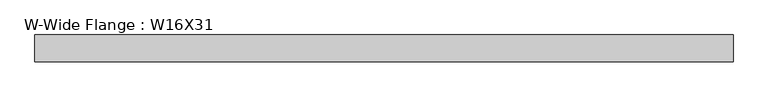
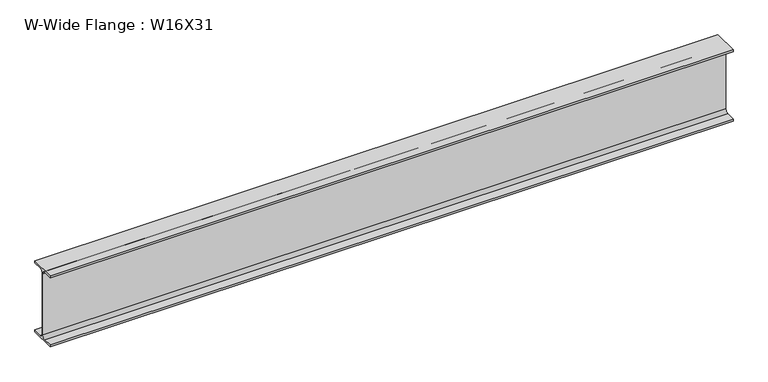
"""IFC4 building model written with IfcOpenShell, lengths in millimetres: beam geometry, W-Wide Flange : W16X31."""

from ifc_helpers import new_model, si_unit, point, frame, frame_2d, origin, place, context, project, spatial, polyline, circle_curve, trimmed, segment, composite_curve, outline, extrude, source, transform, mapped, element, save


def w_wide_flange_w16x31_a2bf4235(model_context):
    return source(origin(), model_context, "Body", "SweptSolid", [
        extrude(outline(composite_curve([segment(polyline([(70.231, -190.754), (70.231, -201.93), (-70.231, -201.93), (-70.231, -190.754), (-20.8915, -190.754)]), True, "CONTINUOUS"), segment(trimmed(circle_curve(frame_2d((-20.8915, -173.355)), 17.399), [point((-20.8915, -190.754))], [point((-3.4925, -173.355))], True, "CARTESIAN"), True, "CONTINUOUS"), segment(polyline([(-3.4925, -173.355), (-3.4925, 173.355)]), True, "CONTINUOUS"), segment(trimmed(circle_curve(frame_2d((-20.8915, 173.355)), 17.399), [point((-3.4925, 173.355))], [point((-20.8915, 190.754))], True, "CARTESIAN"), True, "CONTINUOUS"), segment(polyline([(-20.8915, 190.754), (-70.231, 190.754), (-70.231, 201.93), (70.231, 201.93), (70.231, 190.754), (20.8915, 190.754)]), True, "CONTINUOUS"), segment(trimmed(circle_curve(frame_2d((20.8915, 173.355)), 17.399), [point((20.8915, 190.754))], [point((3.4925, 173.355))], True, "CARTESIAN"), True, "CONTINUOUS"), segment(polyline([(3.4925, 173.355), (3.4925, -173.355)]), True, "CONTINUOUS"), segment(trimmed(circle_curve(frame_2d((20.8915, -173.355)), 17.399), [point((3.4925, -173.355))], [point((20.8915, -190.754))], True, "CARTESIAN"), True, "CONTINUOUS"), segment(polyline([(20.8915, -190.754), (70.231, -190.754)]), True, "CONTINUOUS")], self_intersect=False)), frame((-1896.2018432, 0.0, 0.0), z_axis=(1.0, 0.0, 0.0), x_axis=(0.0, 1.0, 0.0)), (0.0, 0.0, 1.0), 3665.4036864),
    ])


if __name__ == "__main__":
    model = new_model("IFC4")
    model_context = context("Model", 3, world=origin())
    ifc_project = project(units=[si_unit("LENGTHUNIT", "METRE", prefix="MILLI")], contexts=[model_context])
    site = spatial("IfcSite", under=ifc_project)
    building = spatial("IfcBuilding", under=site)
    placement = place(None, origin())
    w_wide_flange_w16x31_shape = w_wide_flange_w16x31_a2bf4235(model_context)
    element("IfcBeam", 1, ObjectType="W-Wide Flange : W16X31", at=placement, inside=building, context=model_context, shape_type="MappedRepresentation", body=[
        mapped(w_wide_flange_w16x31_shape, transform((0.0, 0.0, 0.0), x_axis=(1.0, 0.0, 0.0), y_axis=(0.0, 1.0, 0.0), z_axis=(0.0, 0.0, 1.0))),
    ])
    save(model, "model.ifc")

# Revit data of these elements
# Type "W-Wide Flange : W16X31"
#   Assembly Code = "B10"
#   W = 31
#   Length [instance default] = 5' - 0"
#   bf = 0' - 5.53"
#   d = 1' - 3.9"
#   k = 0' - 1 1/8"
#   k2 = 0' - 0.685"
#   tf = 0' - 0.44"
#   tw = 0' - 0.275"
#   A = 0.0634028 SF
#   Structural Material [instance default] = Steel ASTM A992
# Element 1 (IfcBeam, "W-Wide Flange : W16X31")
#   Structural Material = Steel ASTM A36
#   Materials on its faces: "Steel ASTM A36"
# Materials
#   "Steel ASTM A992": class "Metal", colour RGB 199 199 199, transparency 0, Description = "Structural steel 50ksi", Cost = 0
#   "Steel ASTM A36": class "Metal", colour RGB 199 199 199, transparency 0, Description = "Structural steel, ASTM A36 Grade B, mill finish", Cost = 0
